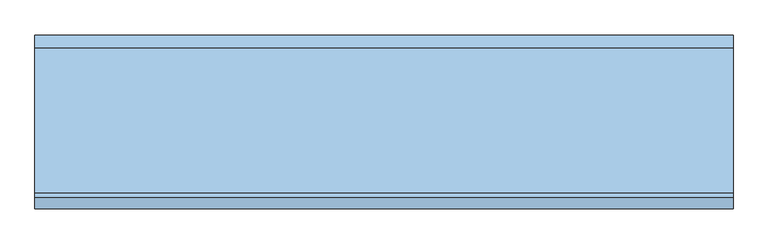
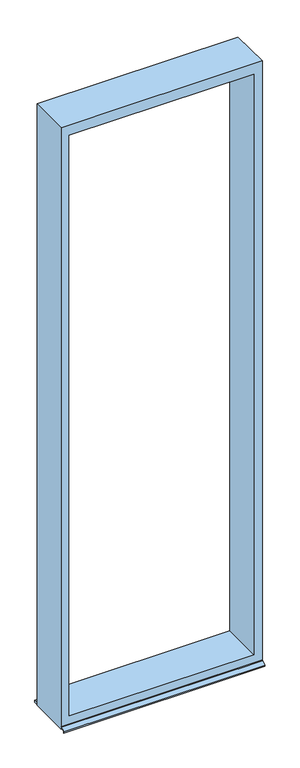
"""IFC4 building model written with IfcOpenShell, lengths in millimetres: window geometry, Fenster - Festverglasung : Feste Verglasung 4.58 x 1.45 3."""

from ifc_helpers import new_model, si_unit, frame, origin, place, context, project, spatial, polyline, outline, extrude, source, transform, mapped, element, save


def window_e8196d3a(model_context):
    return source(origin(), model_context, "Body", "SweptSolid", [
        extrude(outline(polyline([(5580.0, 725.0), (5580.0, -725.0), (1000.0, -725.0), (1000.0, 725.0), (5580.0, 725.0)]), holes=[polyline([(5500.0, 665.0), (1080.0, 665.0), (1080.0, -665.0), (5500.0, -665.0), (5500.0, 665.0)])]), frame((0.0, -147.5214598, 0.0), z_axis=(0.0, 1.0, 0.0), x_axis=(0.0, 0.0, 1.0)), (0.0, 0.0, 1.0), 300.0),
        extrude(outline(polyline([(-725.0, 180.0), (725.0, 180.0), (725.0, 152.4785402), (-725.0, 152.4785402), (-725.0, 180.0)])), frame((0.0, 0.0, 1005.0), z_axis=(0.0, 0.0, 1.0), x_axis=(1.0, 0.0, 0.0)), (0.0, 0.0, 1.0), 15.0),
        extrude(outline(polyline([(-157.5436142, 1020.0), (-147.5214598, 1020.0), (-147.5214598, 1018.0), (-157.3455321, 1018.0), (-178.0, 998.3604634), (-178.0, 990.0), (-180.0, 990.0), (-180.0, 1000.0), (-157.5436142, 1020.0)])), frame((-725.0, 0.0, 0.0), z_axis=(1.0, 0.0, 0.0), x_axis=(0.0, 1.0, 0.0)), (0.0, 0.0, 1.0), 1450.0),
    ])


if __name__ == "__main__":
    model = new_model("IFC4")
    model_context = context("Model", 3, world=origin())
    ifc_project = project(units=[si_unit("LENGTHUNIT", "METRE", prefix="MILLI")], contexts=[model_context])
    site = spatial("IfcSite", under=ifc_project)
    building = spatial("IfcBuilding", under=site)
    placement = place(None, origin())
    window_shape = window_e8196d3a(model_context)
    element("IfcWindow", 1, ObjectType="Fenster - Festverglasung : Feste Verglasung 4.58 x 1.45 3", at=placement, inside=building, context=model_context, shape_type="MappedRepresentation", body=[
        mapped(window_shape, transform((0.0, 0.0, 0.0), x_axis=(1.0, 0.0, 0.0), y_axis=(0.0, 1.0, 0.0), z_axis=(0.0, 0.0, 1.0))),
    ])
    save(model, "model.ifc")

# Revit data of these elements
# Type "Fenster - Festverglasung : Feste Verglasung 4.58 x 1.45 3"
#   Type Mark = "71"
#   Operation = "SinglePanel"
#   Keynote = "16.05.01"
#   Visual Light Transmittance = 0.9
#   Solar Heat Gain Coefficient = 0.78
#   Rough Width = 1.450 m
#   Rough Height = 4.580 m
#   Heat Transfer Coefficient (U) = 3.6886 W/(m²·K)
#   Rahmentiefe = 0.300 m
#   Rahmenhöhe unten = 0.080 m
#   Höhe oberer  Rahmen = 0.080 m
#   Rahmenbreite = 0.060 m
#   Height = 4.580 m
#   Einbautiefe (von außen) [instance default] = 0.080 m
#   Width = 1.450 m
#   Wall Closure = 3
#   Bild [instance default] = none
#   Glas [instance default] = none
#   Innere Fensterbank [instance default] = none
#   Äußere Fensterbank [instance default] = none
#   Construction Type Id = ""
#   Analytic Construction = (empty or 0)
# Element 1 (IfcWindow, "Fenster - Festverglasung : Feste Verglasung 4.58 x 1.45 3")
#   Einbautiefe (von außen) = 0.002479 m
#   Materials on its faces: "Kunststoff - Weiß", "Holz - Birke"
# Materials
#   "Kunststoff - Weiß": class "Kunststoff", colour RGB 249 249 249, transparency 0, Cost = 0
#   "Holz - Birke": class "Holz", colour RGB 213 164 103, transparency 0, Cost = 0
